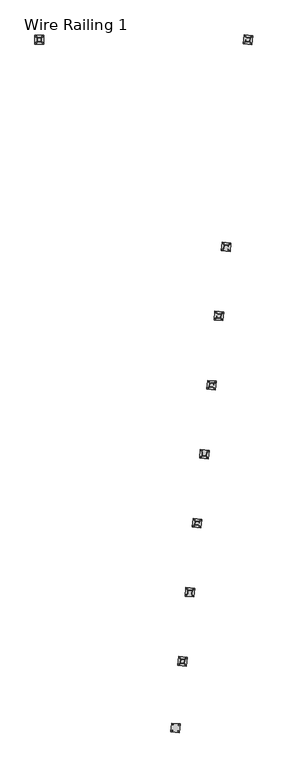
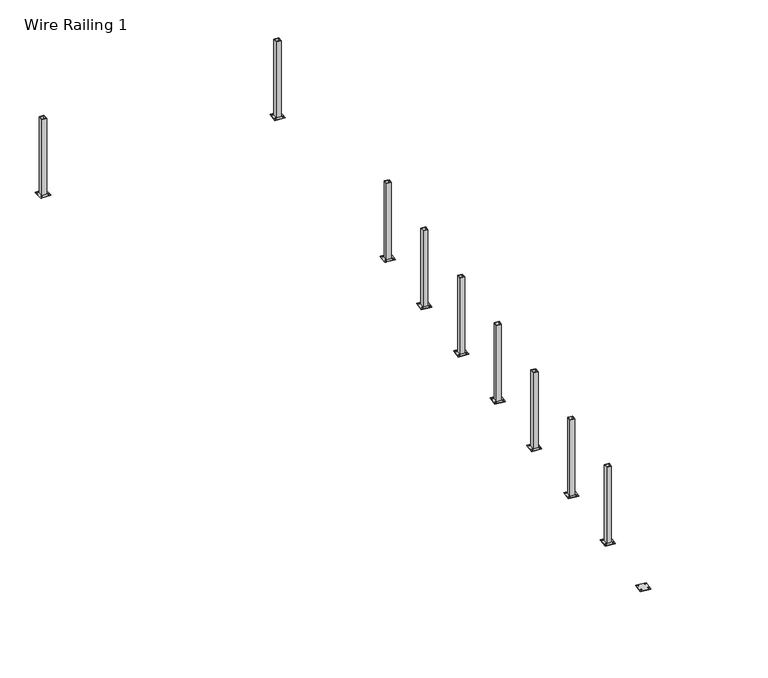
"""IFC4 building model written with IfcOpenShell, lengths in millimetres: railing geometry, Wire Railing 1."""

import ifcopenshell
import ifcopenshell.guid

model = None  # the IFC model being written
_history = None  # IfcOwnerHistory: only IFC2X3 demands one
_inside = {}  # id of a spatial element -> (the spatial element, [elements in it])
_under = {}  # id of a project, library or spatial element -> (it, [spatial elements below it])
_declared = {}  # id of a project -> (the project, [libraries it declares])
_typed = {}  # id of a type object -> (the type object, [elements of that type])
_made_of = {}  # id of a material, layer set ... -> (it, [elements and type objects made of it])


def new_model(schema):
    """Start an empty IFC model of exactly this schema.

    Asked for "IFC4X3", IfcOpenShell would pick the latest addendum, in which some entities
    have other attributes; the version numbers below select the first issue.
    IFC2X3 requires an IfcOwnerHistory on every rooted entity: one is made here for all.
    """
    global model, _history
    if schema == "IFC4X3":
        model = ifcopenshell.file(schema_version=(4, 3, 0, 0))
    else:
        model = ifcopenshell.file(schema=schema)
    _inside.clear()
    _under.clear()
    _declared.clear()
    _typed.clear()
    _made_of.clear()
    _history = None
    if model.schema == "IFC2X3":
        org = make("IfcOrganization", Name="unknown")
        user = make(
            "IfcPersonAndOrganization",
            ThePerson=make("IfcPerson", FamilyName="unknown"),
            TheOrganization=org,
        )
        app = make(
            "IfcApplication",
            ApplicationDeveloper=org,
            Version="unknown",
            ApplicationFullName="unknown",
            ApplicationIdentifier="unknown",
        )
        _history = make(
            "IfcOwnerHistory",
            OwningUser=user,
            OwningApplication=app,
            ChangeAction="ADDED",
            CreationDate=0,
        )
    return model


def make(cls, **values):
    """One entity of the class cls with the attributes given. An attribute that is None is left unset."""
    return model.create_entity(
        cls, **{name: value for name, value in values.items() if value is not None}
    )


def rooted(cls, **values):
    """An entity with a GlobalId (a new one), such as an element, a storey or a relation."""
    return make(cls, GlobalId=ifcopenshell.guid.new(), OwnerHistory=_history, **values)


def si_unit(unit_type, name, prefix=None):
    """IfcSIUnit, for example si_unit("LENGTHUNIT", "METRE", prefix="MILLI")."""
    return make("IfcSIUnit", UnitType=unit_type, Prefix=prefix, Name=name)


def assignment(units):
    """IfcUnitAssignment: the units of a project."""
    return None if units is None else make("IfcUnitAssignment", Units=units)


def point(xyz):
    """IfcCartesianPoint."""
    return None if xyz is None else make("IfcCartesianPoint", Coordinates=xyz)


def direction(xyz):
    """IfcDirection."""
    return None if xyz is None else make("IfcDirection", DirectionRatios=xyz)


def frame(location, z_axis=None, x_axis=None):
    """IfcAxis2Placement3D, a coordinate frame: its origin and axes. An axis left out is left unset."""
    return make(
        "IfcAxis2Placement3D",
        Location=point(location),
        Axis=direction(z_axis),
        RefDirection=direction(x_axis),
    )


def frame_2d(location, x_axis=None):
    """IfcAxis2Placement2D, a coordinate frame in the plane: its origin and x axis."""
    return make(
        "IfcAxis2Placement2D", Location=point(location), RefDirection=direction(x_axis)
    )


def origin():
    """The frame at (0, 0, 0) with its axes left unset."""
    return frame((0.0, 0.0, 0.0))


def place(relative_to, where):
    """IfcLocalPlacement: puts the frame where relative to a parent placement (None: the world)."""
    return make(
        "IfcLocalPlacement", PlacementRelTo=relative_to, RelativePlacement=where
    )


def context(
    kind, dimensions, precision=None, world=None, true_north=None, identifier=None
):
    """IfcGeometricRepresentationContext, for example the 3D "Model" context."""
    return make(
        "IfcGeometricRepresentationContext",
        ContextIdentifier=identifier,
        ContextType=kind,
        CoordinateSpaceDimension=dimensions,
        Precision=precision,
        WorldCoordinateSystem=world,
        TrueNorth=true_north,
    )


def project(units=None, contexts=None):
    """IfcProject with its units and contexts."""
    return rooted(
        "IfcProject",
        Name="project",
        RepresentationContexts=contexts,
        UnitsInContext=assignment(units),
    )


def spatial(cls, under=None, at=None, **own):
    """A site, building, storey or space (cls), placed at a placement, below another one or the project."""
    s = rooted(cls, ObjectPlacement=at, **own)
    if under is not None:
        _under.setdefault(under.id(), (under, []))[1].append(s)
    return s


def polyline(points):
    """IfcPolyline through the points."""
    return make("IfcPolyline", Points=[point(p) for p in points])


def circle_curve(where, radius):
    """IfcCircle in the frame where."""
    return make("IfcCircle", Position=where, Radius=radius)


def trimmed(basis, trim1, trim2, sense, master):
    """IfcTrimmedCurve: the piece of a basis curve between two trims."""
    return make(
        "IfcTrimmedCurve",
        BasisCurve=basis,
        Trim1=trim1,
        Trim2=trim2,
        SenseAgreement=sense,
        MasterRepresentation=master,
    )


def segment(curve, same_sense, transition):
    """IfcCompositeCurveSegment."""
    return make(
        "IfcCompositeCurveSegment",
        Transition=transition,
        SameSense=same_sense,
        ParentCurve=curve,
    )


def composite_curve(segments, self_intersect=None):
    """IfcCompositeCurve: segments joined end to end."""
    return make("IfcCompositeCurve", Segments=segments, SelfIntersect=self_intersect)


def outline(outer, holes=None, kind="AREA"):
    """IfcArbitraryClosedProfileDef: a profile drawn as a closed curve; with holes, ...WithVoids."""
    if holes is None:
        return make("IfcArbitraryClosedProfileDef", ProfileType=kind, OuterCurve=outer)
    return make(
        "IfcArbitraryProfileDefWithVoids",
        ProfileType=kind,
        OuterCurve=outer,
        InnerCurves=holes,
    )


def extrude(swept, where, along, depth):
    """IfcExtrudedAreaSolid: the profile swept, set in the frame where, extruded along a direction by depth."""
    return make(
        "IfcExtrudedAreaSolid",
        SweptArea=swept,
        Position=where,
        ExtrudedDirection=direction(along),
        Depth=depth,
    )


def shape(context_of_items, identifier, shape_type, items):
    """IfcShapeRepresentation: the items that make up one representation, for example the "Body"."""
    return make(
        "IfcShapeRepresentation",
        ContextOfItems=context_of_items,
        RepresentationIdentifier=identifier,
        RepresentationType=shape_type,
        Items=items,
    )


def source(mapping_origin, context_of_items, identifier, shape_type, items):
    """IfcRepresentationMap: a shape defined once, which mapped items show again and again."""
    return make(
        "IfcRepresentationMap",
        MappingOrigin=mapping_origin,
        MappedRepresentation=shape(context_of_items, identifier, shape_type, items),
    )


def transform(
    local_origin,
    x_axis=None,
    y_axis=None,
    z_axis=None,
    scale=None,
    scale2=None,
    scale3=None,
    uniform=True,
):
    """IfcCartesianTransformationOperator3D, or its non-uniform kind. x_axis, y_axis, z_axis: its Axis1, 2, 3."""
    if uniform:
        return make(
            "IfcCartesianTransformationOperator3D",
            Axis1=direction(x_axis),
            Axis2=direction(y_axis),
            LocalOrigin=point(local_origin),
            Scale=scale,
            Axis3=direction(z_axis),
        )
    return make(
        "IfcCartesianTransformationOperator3DnonUniform",
        Axis1=direction(x_axis),
        Axis2=direction(y_axis),
        LocalOrigin=point(local_origin),
        Scale=scale,
        Axis3=direction(z_axis),
        Scale2=scale2,
        Scale3=scale3,
    )


def mapped(mapping_source, mapping_target):
    """IfcMappedItem: shows the shape of a source again, moved by a transform."""
    return make(
        "IfcMappedItem", MappingSource=mapping_source, MappingTarget=mapping_target
    )


def made_of(thing, what):
    """Note that an element or type object is made of a material, layer set ...; save() writes the relation."""
    if what is not None:
        _made_of.setdefault(what.id(), (what, []))[1].append(thing)
    return thing


def element(
    cls,
    number,
    at=None,
    inside=None,
    cuts=None,
    type_object=None,
    material=None,
    context=None,
    identifier="Body",
    shape_type=None,
    held_by="IfcProductDefinitionShape",
    body=None,
    shapes=None,
    **own,
):
    """One element of the class cls, such as IfcWall. Its Tag is "e" and its number.

    at: its placement. inside: the storey or other place that contains it. cuts: it is an
    opening in that element (IfcRelVoidsElement). A single representation is given by context,
    identifier, shape_type and body (its items); several are given by shapes. held_by: the class
    of the entity that holds the representations. save() writes the other relations.
    """
    e = rooted(cls, Tag="e%d" % number, ObjectPlacement=at, **own)
    if body is not None:
        shapes = [shape(context, identifier, shape_type, body)]
    if shapes is not None:
        e.Representation = make(held_by, Representations=shapes)
    if inside is not None:
        _inside.setdefault(inside.id(), (inside, []))[1].append(e)
    if cuts is not None:
        rooted(
            "IfcRelVoidsElement", RelatingBuildingElement=cuts, RelatedOpeningElement=e
        )
    if type_object is not None:
        _typed.setdefault(type_object.id(), (type_object, []))[1].append(e)
    return made_of(e, material)


def aggregate(whole, parts):
    """IfcRelAggregates: a whole, such as a stair, and the parts it consists of."""
    return rooted("IfcRelAggregates", RelatingObject=whole, RelatedObjects=parts)


def save(model, path):
    """Write the relations noted so far, then the file.

    IfcRelAggregates (storeys below a building ...), IfcRelContainedInSpatialStructure (elements
    in a storey), IfcRelDefinesByType, IfcRelAssociatesMaterial and IfcRelDeclares: one each for
    every whole, place, type object, material and project.
    """
    for whole, parts in _under.values():
        aggregate(whole, parts)
    for where, things in _inside.values():
        rooted(
            "IfcRelContainedInSpatialStructure",
            RelatedElements=things,
            RelatingStructure=where,
        )
    for kind, things in _typed.values():
        rooted("IfcRelDefinesByType", RelatedObjects=things, RelatingType=kind)
    for what, things in _made_of.values():
        rooted("IfcRelAssociatesMaterial", RelatedObjects=things, RelatingMaterial=what)
    for by, libraries in _declared.values():
        rooted("IfcRelDeclares", RelatingContext=by, RelatedDefinitions=libraries)
    model.write(path)


def wire_railing_1_b7aef56b(model_context):
    return source(origin(), model_context, "Body", "SweptSolid", [
        extrude(outline(composite_curve([segment(trimmed(circle_curve(frame_2d((34964.0191905, 37829.4240871)), 6.35), [point((34957.7039765, 37830.0878428))], [point((34970.3344045, 37828.7603313))], False, "CARTESIAN"), True, "CONTINUOUS"), segment(trimmed(circle_curve(frame_2d((34964.0191905, 37829.4240871)), 6.35), [point((34970.3344045, 37828.7603313))], [point((34957.7039765, 37830.0878428))], False, "CARTESIAN"), True, "CONTINUOUS")], self_intersect=False)), frame((0.0, 0.0, 269259.05), z_axis=(0.0, 0.0, 1.0), x_axis=(1.0, 0.0, 0.0)), (0.0, 0.0, 1.0), 12.7),
        extrude(outline(composite_curve([segment(trimmed(circle_curve(frame_2d((35052.432187, 37820.1315067)), 6.35), [point((35046.116973, 37820.7952624))], [point((35058.747401, 37819.4677509))], False, "CARTESIAN"), True, "CONTINUOUS"), segment(trimmed(circle_curve(frame_2d((35052.432187, 37820.1315067)), 6.35), [point((35058.747401, 37819.4677509))], [point((35046.116973, 37820.7952624))], False, "CARTESIAN"), True, "CONTINUOUS")], self_intersect=False)), frame((0.0, 0.0, 269259.05), z_axis=(0.0, 0.0, 1.0), x_axis=(1.0, 0.0, 0.0)), (0.0, 0.0, 1.0), 12.7),
        extrude(outline(composite_curve([segment(trimmed(circle_curve(frame_2d((34973.3117709, 37917.8370836)), 6.35), [point((34966.9965569, 37918.5008393))], [point((34979.6269849, 37917.1733278))], False, "CARTESIAN"), True, "CONTINUOUS"), segment(trimmed(circle_curve(frame_2d((34973.3117709, 37917.8370836)), 6.35), [point((34979.6269849, 37917.1733278))], [point((34966.9965569, 37918.5008393))], False, "CARTESIAN"), True, "CONTINUOUS")], self_intersect=False)), frame((0.0, 0.0, 269259.05), z_axis=(0.0, 0.0, 1.0), x_axis=(1.0, 0.0, 0.0)), (0.0, 0.0, 1.0), 12.7),
        extrude(outline(composite_curve([segment(trimmed(circle_curve(frame_2d((35061.7247674, 37908.5445032)), 6.35), [point((35055.4095533, 37909.2082589))], [point((35068.0399814, 37907.8807474))], False, "CARTESIAN"), True, "CONTINUOUS"), segment(trimmed(circle_curve(frame_2d((35061.7247674, 37908.5445032)), 6.35), [point((35068.0399814, 37907.8807474))], [point((35055.4095533, 37909.2082589))], False, "CARTESIAN"), True, "CONTINUOUS")], self_intersect=False)), frame((0.0, 0.0, 269259.05), z_axis=(0.0, 0.0, 1.0), x_axis=(1.0, 0.0, 0.0)), (0.0, 0.0, 1.0), 12.7),
        extrude(outline(polyline([(35069.3865619, 37799.1945973), (34943.0822812, 37812.4697122), (34956.357396, 37938.7739929), (35082.6616767, 37925.498878), (35069.3865619, 37799.1945973)])), frame((0.0, 0.0, 269259.05), z_axis=(0.0, 0.0, 1.0), x_axis=(1.0, 0.0, 0.0)), (0.0, 0.0, 1.0), 6.35),
        extrude(outline(polyline([(35039.7164058, 37835.8341887), (34979.7218725, 37842.1398682), (34986.027552, 37902.1344016), (35046.0220854, 37895.828722), (35039.7164058, 37835.8341887)]), holes=[polyline([(35034.0649475, 37842.8131584), (35039.0431156, 37890.1772637), (34991.6790103, 37895.1554318), (34986.7008423, 37847.7913265), (35034.0649475, 37842.8131584)])]), frame((0.0, 0.0, 269259.05), z_axis=(0.0, 0.0, 1.0), x_axis=(1.0, 0.0, 0.0)), (0.0, 0.0, 1.0), 1047.75),
        extrude(outline(composite_curve([segment(trimmed(circle_curve(frame_2d((34858.2648202, 36823.238465)), 6.35), [point((34851.9496061, 36823.9022208))], [point((34864.5800342, 36822.5747093))], False, "CARTESIAN"), True, "CONTINUOUS"), segment(trimmed(circle_curve(frame_2d((34858.2648202, 36823.238465)), 6.35), [point((34864.5800342, 36822.5747093))], [point((34851.9496061, 36823.9022208))], False, "CARTESIAN"), True, "CONTINUOUS")], self_intersect=False)), frame((0.0, 0.0, 269259.05), z_axis=(0.0, 0.0, 1.0), x_axis=(1.0, 0.0, 0.0)), (0.0, 0.0, 1.0), 12.7),
        extrude(outline(composite_curve([segment(trimmed(circle_curve(frame_2d((34946.6778167, 36813.9458846)), 6.35), [point((34940.3626026, 36814.6096404))], [point((34952.9930307, 36813.2821289))], False, "CARTESIAN"), True, "CONTINUOUS"), segment(trimmed(circle_curve(frame_2d((34946.6778167, 36813.9458846)), 6.35), [point((34952.9930307, 36813.2821289))], [point((34940.3626026, 36814.6096404))], False, "CARTESIAN"), True, "CONTINUOUS")], self_intersect=False)), frame((0.0, 0.0, 269259.05), z_axis=(0.0, 0.0, 1.0), x_axis=(1.0, 0.0, 0.0)), (0.0, 0.0, 1.0), 12.7),
        extrude(outline(composite_curve([segment(trimmed(circle_curve(frame_2d((34867.5574005, 36911.6514615)), 6.35), [point((34861.2421865, 36912.3152173))], [point((34873.8726146, 36910.9877058))], False, "CARTESIAN"), True, "CONTINUOUS"), segment(trimmed(circle_curve(frame_2d((34867.5574005, 36911.6514615)), 6.35), [point((34873.8726146, 36910.9877058))], [point((34861.2421865, 36912.3152173))], False, "CARTESIAN"), True, "CONTINUOUS")], self_intersect=False)), frame((0.0, 0.0, 269259.05), z_axis=(0.0, 0.0, 1.0), x_axis=(1.0, 0.0, 0.0)), (0.0, 0.0, 1.0), 12.7),
        extrude(outline(composite_curve([segment(trimmed(circle_curve(frame_2d((34955.970397, 36902.3588811)), 6.35), [point((34949.655183, 36903.0226369))], [point((34962.2856111, 36901.6951254))], False, "CARTESIAN"), True, "CONTINUOUS"), segment(trimmed(circle_curve(frame_2d((34955.970397, 36902.3588811)), 6.35), [point((34962.2856111, 36901.6951254))], [point((34949.655183, 36903.0226369))], False, "CARTESIAN"), True, "CONTINUOUS")], self_intersect=False)), frame((0.0, 0.0, 269259.05), z_axis=(0.0, 0.0, 1.0), x_axis=(1.0, 0.0, 0.0)), (0.0, 0.0, 1.0), 12.7),
        extrude(outline(polyline([(34963.6321915, 36793.0089753), (34837.3279108, 36806.2840901), (34850.6030257, 36932.5883709), (34976.9073064, 36919.313256), (34963.6321915, 36793.0089753)])), frame((0.0, 0.0, 269259.05), z_axis=(0.0, 0.0, 1.0), x_axis=(1.0, 0.0, 0.0)), (0.0, 0.0, 1.0), 6.35),
        extrude(outline(polyline([(34933.9620355, 36829.6485666), (34873.9675022, 36835.9542462), (34880.2731817, 36895.9487795), (34940.267715, 36889.6431), (34933.9620355, 36829.6485666)]), holes=[polyline([(34928.3105772, 36836.6275364), (34933.2887453, 36883.9916417), (34885.92464, 36888.9698097), (34880.9464719, 36841.6057045), (34928.3105772, 36836.6275364)])]), frame((0.0, 0.0, 269259.05), z_axis=(0.0, 0.0, 1.0), x_axis=(1.0, 0.0, 0.0)), (0.0, 0.0, 1.0), 1047.75),
        extrude(outline(composite_curve([segment(trimmed(circle_curve(frame_2d((34752.5104498, 35817.052843)), 6.35), [point((34746.1952358, 35817.7165987))], [point((34758.8256639, 35816.3890873))], False, "CARTESIAN"), True, "CONTINUOUS"), segment(trimmed(circle_curve(frame_2d((34752.5104498, 35817.052843)), 6.35), [point((34758.8256639, 35816.3890873))], [point((34746.1952358, 35817.7165987))], False, "CARTESIAN"), True, "CONTINUOUS")], self_intersect=False)), frame((0.0, 0.0, 269259.05), z_axis=(0.0, 0.0, 1.0), x_axis=(1.0, 0.0, 0.0)), (0.0, 0.0, 1.0), 12.7),
        extrude(outline(composite_curve([segment(trimmed(circle_curve(frame_2d((34840.9234463, 35807.7602626)), 6.35), [point((34834.6082323, 35808.4240184))], [point((34847.2386604, 35807.0965069))], False, "CARTESIAN"), True, "CONTINUOUS"), segment(trimmed(circle_curve(frame_2d((34840.9234463, 35807.7602626)), 6.35), [point((34847.2386604, 35807.0965069))], [point((34834.6082323, 35808.4240184))], False, "CARTESIAN"), True, "CONTINUOUS")], self_intersect=False)), frame((0.0, 0.0, 269259.05), z_axis=(0.0, 0.0, 1.0), x_axis=(1.0, 0.0, 0.0)), (0.0, 0.0, 1.0), 12.7),
        extrude(outline(composite_curve([segment(trimmed(circle_curve(frame_2d((34761.8030302, 35905.4658395)), 6.35), [point((34755.4878162, 35906.1295952))], [point((34768.1182442, 35904.8020838))], False, "CARTESIAN"), True, "CONTINUOUS"), segment(trimmed(circle_curve(frame_2d((34761.8030302, 35905.4658395)), 6.35), [point((34768.1182442, 35904.8020838))], [point((34755.4878162, 35906.1295952))], False, "CARTESIAN"), True, "CONTINUOUS")], self_intersect=False)), frame((0.0, 0.0, 269259.05), z_axis=(0.0, 0.0, 1.0), x_axis=(1.0, 0.0, 0.0)), (0.0, 0.0, 1.0), 12.7),
        extrude(outline(composite_curve([segment(trimmed(circle_curve(frame_2d((34850.2160267, 35896.1732591)), 6.35), [point((34843.9008127, 35896.8370148))], [point((34856.5312407, 35895.5095034))], False, "CARTESIAN"), True, "CONTINUOUS"), segment(trimmed(circle_curve(frame_2d((34850.2160267, 35896.1732591)), 6.35), [point((34856.5312407, 35895.5095034))], [point((34843.9008127, 35896.8370148))], False, "CARTESIAN"), True, "CONTINUOUS")], self_intersect=False)), frame((0.0, 0.0, 269259.05), z_axis=(0.0, 0.0, 1.0), x_axis=(1.0, 0.0, 0.0)), (0.0, 0.0, 1.0), 12.7),
        extrude(outline(polyline([(34857.8778212, 35786.8233533), (34731.5735405, 35800.0984681), (34744.8486553, 35926.4027488), (34871.152936, 35913.127634), (34857.8778212, 35786.8233533)])), frame((0.0, 0.0, 269259.05), z_axis=(0.0, 0.0, 1.0), x_axis=(1.0, 0.0, 0.0)), (0.0, 0.0, 1.0), 6.35),
        extrude(outline(polyline([(34828.2076652, 35823.4629446), (34768.2131318, 35829.7686242), (34774.5188114, 35889.7631575), (34834.5133447, 35883.4574779), (34828.2076652, 35823.4629446)]), holes=[polyline([(34822.5562069, 35830.4419144), (34827.5343749, 35877.8060197), (34780.1702697, 35882.7841877), (34775.1921016, 35835.4200824), (34822.5562069, 35830.4419144)])]), frame((0.0, 0.0, 269259.05), z_axis=(0.0, 0.0, 1.0), x_axis=(1.0, 0.0, 0.0)), (0.0, 0.0, 1.0), 1047.75),
        extrude(outline(composite_curve([segment(trimmed(circle_curve(frame_2d((34646.7560795, 34810.867221)), 6.35), [point((34640.4408654, 34811.5309767))], [point((34653.0712935, 34810.2034652))], False, "CARTESIAN"), True, "CONTINUOUS"), segment(trimmed(circle_curve(frame_2d((34646.7560795, 34810.867221)), 6.35), [point((34653.0712935, 34810.2034652))], [point((34640.4408654, 34811.5309767))], False, "CARTESIAN"), True, "CONTINUOUS")], self_intersect=False)), frame((0.0, 0.0, 269259.05), z_axis=(0.0, 0.0, 1.0), x_axis=(1.0, 0.0, 0.0)), (0.0, 0.0, 1.0), 12.7),
        extrude(outline(composite_curve([segment(trimmed(circle_curve(frame_2d((34735.169076, 34801.5746406)), 6.35), [point((34728.8538619, 34802.2383963))], [point((34741.48429, 34800.9108848))], False, "CARTESIAN"), True, "CONTINUOUS"), segment(trimmed(circle_curve(frame_2d((34735.169076, 34801.5746406)), 6.35), [point((34741.48429, 34800.9108848))], [point((34728.8538619, 34802.2383963))], False, "CARTESIAN"), True, "CONTINUOUS")], self_intersect=False)), frame((0.0, 0.0, 269259.05), z_axis=(0.0, 0.0, 1.0), x_axis=(1.0, 0.0, 0.0)), (0.0, 0.0, 1.0), 12.7),
        extrude(outline(composite_curve([segment(trimmed(circle_curve(frame_2d((34656.0486599, 34899.2802175)), 6.35), [point((34649.7334458, 34899.9439732))], [point((34662.3638739, 34898.6164617))], False, "CARTESIAN"), True, "CONTINUOUS"), segment(trimmed(circle_curve(frame_2d((34656.0486599, 34899.2802175)), 6.35), [point((34662.3638739, 34898.6164617))], [point((34649.7334458, 34899.9439732))], False, "CARTESIAN"), True, "CONTINUOUS")], self_intersect=False)), frame((0.0, 0.0, 269259.05), z_axis=(0.0, 0.0, 1.0), x_axis=(1.0, 0.0, 0.0)), (0.0, 0.0, 1.0), 12.7),
        extrude(outline(composite_curve([segment(trimmed(circle_curve(frame_2d((34744.4616564, 34889.9876371)), 6.35), [point((34738.1464423, 34890.6513928))], [point((34750.7768704, 34889.3238813))], False, "CARTESIAN"), True, "CONTINUOUS"), segment(trimmed(circle_curve(frame_2d((34744.4616564, 34889.9876371)), 6.35), [point((34750.7768704, 34889.3238813))], [point((34738.1464423, 34890.6513928))], False, "CARTESIAN"), True, "CONTINUOUS")], self_intersect=False)), frame((0.0, 0.0, 269259.05), z_axis=(0.0, 0.0, 1.0), x_axis=(1.0, 0.0, 0.0)), (0.0, 0.0, 1.0), 12.7),
        extrude(outline(polyline([(34752.1234509, 34780.6377312), (34625.8191702, 34793.9128461), (34639.094285, 34920.2171268), (34765.3985657, 34906.942012), (34752.1234509, 34780.6377312)])), frame((0.0, 0.0, 269259.05), z_axis=(0.0, 0.0, 1.0), x_axis=(1.0, 0.0, 0.0)), (0.0, 0.0, 1.0), 6.35),
        extrude(outline(polyline([(34722.4532948, 34817.2773226), (34662.4587615, 34823.5830021), (34668.764441, 34883.5775355), (34728.7589744, 34877.2718559), (34722.4532948, 34817.2773226)]), holes=[polyline([(34716.8018365, 34824.2562924), (34721.7800046, 34871.6203976), (34674.4158993, 34876.5985657), (34669.4377313, 34829.2344604), (34716.8018365, 34824.2562924)])]), frame((0.0, 0.0, 269259.05), z_axis=(0.0, 0.0, 1.0), x_axis=(1.0, 0.0, 0.0)), (0.0, 0.0, 1.0), 1047.75),
        extrude(outline(composite_curve([segment(trimmed(circle_curve(frame_2d((34541.0017091, 33804.6815989)), 6.35), [point((34534.6864951, 33805.3453547))], [point((34547.3169232, 33804.0178432))], False, "CARTESIAN"), True, "CONTINUOUS"), segment(trimmed(circle_curve(frame_2d((34541.0017091, 33804.6815989)), 6.35), [point((34547.3169232, 33804.0178432))], [point((34534.6864951, 33805.3453547))], False, "CARTESIAN"), True, "CONTINUOUS")], self_intersect=False)), frame((0.0, 0.0, 269259.05), z_axis=(0.0, 0.0, 1.0), x_axis=(1.0, 0.0, 0.0)), (0.0, 0.0, 1.0), 12.7),
        extrude(outline(composite_curve([segment(trimmed(circle_curve(frame_2d((34629.4147056, 33795.3890186)), 6.35), [point((34623.0994916, 33796.0527743))], [point((34635.7299197, 33794.7252628))], False, "CARTESIAN"), True, "CONTINUOUS"), segment(trimmed(circle_curve(frame_2d((34629.4147056, 33795.3890186)), 6.35), [point((34635.7299197, 33794.7252628))], [point((34623.0994916, 33796.0527743))], False, "CARTESIAN"), True, "CONTINUOUS")], self_intersect=False)), frame((0.0, 0.0, 269259.05), z_axis=(0.0, 0.0, 1.0), x_axis=(1.0, 0.0, 0.0)), (0.0, 0.0, 1.0), 12.7),
        extrude(outline(composite_curve([segment(trimmed(circle_curve(frame_2d((34550.2942895, 33893.0945954)), 6.35), [point((34543.9790755, 33893.7583512))], [point((34556.6095036, 33892.4308397))], False, "CARTESIAN"), True, "CONTINUOUS"), segment(trimmed(circle_curve(frame_2d((34550.2942895, 33893.0945954)), 6.35), [point((34556.6095036, 33892.4308397))], [point((34543.9790755, 33893.7583512))], False, "CARTESIAN"), True, "CONTINUOUS")], self_intersect=False)), frame((0.0, 0.0, 269259.05), z_axis=(0.0, 0.0, 1.0), x_axis=(1.0, 0.0, 0.0)), (0.0, 0.0, 1.0), 12.7),
        extrude(outline(composite_curve([segment(trimmed(circle_curve(frame_2d((34638.707286, 33883.802015)), 6.35), [point((34632.392072, 33884.4657708))], [point((34645.0225001, 33883.1382593))], False, "CARTESIAN"), True, "CONTINUOUS"), segment(trimmed(circle_curve(frame_2d((34638.707286, 33883.802015)), 6.35), [point((34645.0225001, 33883.1382593))], [point((34632.392072, 33884.4657708))], False, "CARTESIAN"), True, "CONTINUOUS")], self_intersect=False)), frame((0.0, 0.0, 269259.05), z_axis=(0.0, 0.0, 1.0), x_axis=(1.0, 0.0, 0.0)), (0.0, 0.0, 1.0), 12.7),
        extrude(outline(polyline([(34646.3690805, 33774.4521092), (34520.0647998, 33787.7272241), (34533.3399146, 33914.0315048), (34659.6441954, 33900.7563899), (34646.3690805, 33774.4521092)])), frame((0.0, 0.0, 269259.05), z_axis=(0.0, 0.0, 1.0), x_axis=(1.0, 0.0, 0.0)), (0.0, 0.0, 1.0), 6.35),
        extrude(outline(polyline([(34616.6989245, 33811.0917005), (34556.7043911, 33817.3973801), (34563.0100707, 33877.3919134), (34623.004604, 33871.0862339), (34616.6989245, 33811.0917005)]), holes=[polyline([(34611.0474662, 33818.0706703), (34616.0256343, 33865.4347756), (34568.661529, 33870.4129437), (34563.6833609, 33823.0488384), (34611.0474662, 33818.0706703)])]), frame((0.0, 0.0, 269259.05), z_axis=(0.0, 0.0, 1.0), x_axis=(1.0, 0.0, 0.0)), (0.0, 0.0, 1.0), 1047.75),
        extrude(outline(composite_curve([segment(trimmed(circle_curve(frame_2d((34435.2473388, 32798.4959769)), 6.35), [point((34428.9321248, 32799.1597326))], [point((34441.5625528, 32797.8322212))], False, "CARTESIAN"), True, "CONTINUOUS"), segment(trimmed(circle_curve(frame_2d((34435.2473388, 32798.4959769)), 6.35), [point((34441.5625528, 32797.8322212))], [point((34428.9321248, 32799.1597326))], False, "CARTESIAN"), True, "CONTINUOUS")], self_intersect=False)), frame((0.0, 0.0, 269259.05), z_axis=(0.0, 0.0, 1.0), x_axis=(1.0, 0.0, 0.0)), (0.0, 0.0, 1.0), 12.7),
        extrude(outline(composite_curve([segment(trimmed(circle_curve(frame_2d((34523.6603353, 32789.2033965)), 6.35), [point((34517.3451213, 32789.8671523))], [point((34529.9755493, 32788.5396408))], False, "CARTESIAN"), True, "CONTINUOUS"), segment(trimmed(circle_curve(frame_2d((34523.6603353, 32789.2033965)), 6.35), [point((34529.9755493, 32788.5396408))], [point((34517.3451213, 32789.8671523))], False, "CARTESIAN"), True, "CONTINUOUS")], self_intersect=False)), frame((0.0, 0.0, 269259.05), z_axis=(0.0, 0.0, 1.0), x_axis=(1.0, 0.0, 0.0)), (0.0, 0.0, 1.0), 12.7),
        extrude(outline(composite_curve([segment(trimmed(circle_curve(frame_2d((34444.5399192, 32886.9089734)), 6.35), [point((34438.2247052, 32887.5727291))], [point((34450.8551332, 32886.2452177))], False, "CARTESIAN"), True, "CONTINUOUS"), segment(trimmed(circle_curve(frame_2d((34444.5399192, 32886.9089734)), 6.35), [point((34450.8551332, 32886.2452177))], [point((34438.2247052, 32887.5727291))], False, "CARTESIAN"), True, "CONTINUOUS")], self_intersect=False)), frame((0.0, 0.0, 269259.05), z_axis=(0.0, 0.0, 1.0), x_axis=(1.0, 0.0, 0.0)), (0.0, 0.0, 1.0), 12.7),
        extrude(outline(composite_curve([segment(trimmed(circle_curve(frame_2d((34532.9529157, 32877.616393)), 6.35), [point((34526.6377017, 32878.2801488))], [point((34539.2681297, 32876.9526373))], False, "CARTESIAN"), True, "CONTINUOUS"), segment(trimmed(circle_curve(frame_2d((34532.9529157, 32877.616393)), 6.35), [point((34539.2681297, 32876.9526373))], [point((34526.6377017, 32878.2801488))], False, "CARTESIAN"), True, "CONTINUOUS")], self_intersect=False)), frame((0.0, 0.0, 269259.05), z_axis=(0.0, 0.0, 1.0), x_axis=(1.0, 0.0, 0.0)), (0.0, 0.0, 1.0), 12.7),
        extrude(outline(polyline([(34540.6147102, 32768.2664872), (34414.3104295, 32781.541602), (34427.5855443, 32907.8458827), (34553.889825, 32894.5707679), (34540.6147102, 32768.2664872)])), frame((0.0, 0.0, 269259.05), z_axis=(0.0, 0.0, 1.0), x_axis=(1.0, 0.0, 0.0)), (0.0, 0.0, 1.0), 6.35),
        extrude(outline(polyline([(34510.9445541, 32804.9060785), (34450.9500208, 32811.2117581), (34457.2557004, 32871.2062914), (34517.2502337, 32864.9006119), (34510.9445541, 32804.9060785)]), holes=[polyline([(34505.2930959, 32811.8850483), (34510.2712639, 32859.2491536), (34462.9071586, 32864.2273216), (34457.9289906, 32816.8632164), (34505.2930959, 32811.8850483)])]), frame((0.0, 0.0, 269259.05), z_axis=(0.0, 0.0, 1.0), x_axis=(1.0, 0.0, 0.0)), (0.0, 0.0, 1.0), 1047.75),
        extrude(outline(composite_curve([segment(trimmed(circle_curve(frame_2d((34329.4929685, 31792.3103549)), 6.35), [point((34323.1777544, 31792.9741106))], [point((34335.8081825, 31791.6465991))], False, "CARTESIAN"), True, "CONTINUOUS"), segment(trimmed(circle_curve(frame_2d((34329.4929685, 31792.3103549)), 6.35), [point((34335.8081825, 31791.6465991))], [point((34323.1777544, 31792.9741106))], False, "CARTESIAN"), True, "CONTINUOUS")], self_intersect=False)), frame((0.0, 0.0, 269259.05), z_axis=(0.0, 0.0, 1.0), x_axis=(1.0, 0.0, 0.0)), (0.0, 0.0, 1.0), 12.7),
        extrude(outline(composite_curve([segment(trimmed(circle_curve(frame_2d((34417.905965, 31783.0177745)), 6.35), [point((34411.5907509, 31783.6815302))], [point((34424.221179, 31782.3540188))], False, "CARTESIAN"), True, "CONTINUOUS"), segment(trimmed(circle_curve(frame_2d((34417.905965, 31783.0177745)), 6.35), [point((34424.221179, 31782.3540188))], [point((34411.5907509, 31783.6815302))], False, "CARTESIAN"), True, "CONTINUOUS")], self_intersect=False)), frame((0.0, 0.0, 269259.05), z_axis=(0.0, 0.0, 1.0), x_axis=(1.0, 0.0, 0.0)), (0.0, 0.0, 1.0), 12.7),
        extrude(outline(composite_curve([segment(trimmed(circle_curve(frame_2d((34338.7855489, 31880.7233514)), 6.35), [point((34332.4703348, 31881.3871071))], [point((34345.1007629, 31880.0595956))], False, "CARTESIAN"), True, "CONTINUOUS"), segment(trimmed(circle_curve(frame_2d((34338.7855489, 31880.7233514)), 6.35), [point((34345.1007629, 31880.0595956))], [point((34332.4703348, 31881.3871071))], False, "CARTESIAN"), True, "CONTINUOUS")], self_intersect=False)), frame((0.0, 0.0, 269259.05), z_axis=(0.0, 0.0, 1.0), x_axis=(1.0, 0.0, 0.0)), (0.0, 0.0, 1.0), 12.7),
        extrude(outline(composite_curve([segment(trimmed(circle_curve(frame_2d((34427.1985454, 31871.430771)), 6.35), [point((34420.8833313, 31872.0945267))], [point((34433.5137594, 31870.7670152))], False, "CARTESIAN"), True, "CONTINUOUS"), segment(trimmed(circle_curve(frame_2d((34427.1985454, 31871.430771)), 6.35), [point((34433.5137594, 31870.7670152))], [point((34420.8833313, 31872.0945267))], False, "CARTESIAN"), True, "CONTINUOUS")], self_intersect=False)), frame((0.0, 0.0, 269259.05), z_axis=(0.0, 0.0, 1.0), x_axis=(1.0, 0.0, 0.0)), (0.0, 0.0, 1.0), 12.7),
        extrude(outline(polyline([(34434.8603398, 31762.0808652), (34308.5560591, 31775.35598), (34321.831174, 31901.6602607), (34448.1354547, 31888.3851459), (34434.8603398, 31762.0808652)])), frame((0.0, 0.0, 269259.05), z_axis=(0.0, 0.0, 1.0), x_axis=(1.0, 0.0, 0.0)), (0.0, 0.0, 1.0), 6.35),
        extrude(outline(polyline([(34405.1901838, 31798.7204565), (34345.1956505, 31805.026136), (34351.50133, 31865.0206694), (34411.4958634, 31858.7149898), (34405.1901838, 31798.7204565)]), holes=[polyline([(34399.5387255, 31805.6994263), (34404.5168936, 31853.0635315), (34357.1527883, 31858.0416996), (34352.1746202, 31810.6775943), (34399.5387255, 31805.6994263)])]), frame((0.0, 0.0, 269259.05), z_axis=(0.0, 0.0, 1.0), x_axis=(1.0, 0.0, 0.0)), (0.0, 0.0, 1.0), 1047.75),
        extrude(outline(composite_curve([segment(trimmed(circle_curve(frame_2d((35281.2823015, 40847.9809531)), 6.35), [point((35274.9670875, 40848.6447089))], [point((35287.5975156, 40847.3171974))], False, "CARTESIAN"), True, "CONTINUOUS"), segment(trimmed(circle_curve(frame_2d((35281.2823015, 40847.9809531)), 6.35), [point((35287.5975156, 40847.3171974))], [point((35274.9670875, 40848.6447089))], False, "CARTESIAN"), True, "CONTINUOUS")], self_intersect=False)), frame((0.0, 0.0, 269259.05), z_axis=(0.0, 0.0, 1.0), x_axis=(1.0, 0.0, 0.0)), (0.0, 0.0, 1.0), 12.7),
        extrude(outline(composite_curve([segment(trimmed(circle_curve(frame_2d((35369.695298, 40838.6883728)), 6.35), [point((35363.380084, 40839.3521285))], [point((35376.0105121, 40838.024617))], False, "CARTESIAN"), True, "CONTINUOUS"), segment(trimmed(circle_curve(frame_2d((35369.695298, 40838.6883728)), 6.35), [point((35376.0105121, 40838.024617))], [point((35363.380084, 40839.3521285))], False, "CARTESIAN"), True, "CONTINUOUS")], self_intersect=False)), frame((0.0, 0.0, 269259.05), z_axis=(0.0, 0.0, 1.0), x_axis=(1.0, 0.0, 0.0)), (0.0, 0.0, 1.0), 12.7),
        extrude(outline(composite_curve([segment(trimmed(circle_curve(frame_2d((35290.5748819, 40936.3939496)), 6.35), [point((35284.2596679, 40937.0577054))], [point((35296.8900959, 40935.7301939))], False, "CARTESIAN"), True, "CONTINUOUS"), segment(trimmed(circle_curve(frame_2d((35290.5748819, 40936.3939496)), 6.35), [point((35296.8900959, 40935.7301939))], [point((35284.2596679, 40937.0577054))], False, "CARTESIAN"), True, "CONTINUOUS")], self_intersect=False)), frame((0.0, 0.0, 269259.05), z_axis=(0.0, 0.0, 1.0), x_axis=(1.0, 0.0, 0.0)), (0.0, 0.0, 1.0), 12.7),
        extrude(outline(composite_curve([segment(trimmed(circle_curve(frame_2d((35378.9878784, 40927.1013693)), 6.35), [point((35372.6726644, 40927.765125))], [point((35385.3030924, 40926.4376135))], False, "CARTESIAN"), True, "CONTINUOUS"), segment(trimmed(circle_curve(frame_2d((35378.9878784, 40927.1013693)), 6.35), [point((35385.3030924, 40926.4376135))], [point((35372.6726644, 40927.765125))], False, "CARTESIAN"), True, "CONTINUOUS")], self_intersect=False)), frame((0.0, 0.0, 269259.05), z_axis=(0.0, 0.0, 1.0), x_axis=(1.0, 0.0, 0.0)), (0.0, 0.0, 1.0), 12.7),
        extrude(outline(polyline([(35386.6496729, 40817.7514634), (35260.3453922, 40831.0265783), (35273.620507, 40957.330859), (35399.9247877, 40944.0557441), (35386.6496729, 40817.7514634)])), frame((0.0, 0.0, 269259.05), z_axis=(0.0, 0.0, 1.0), x_axis=(1.0, 0.0, 0.0)), (0.0, 0.0, 1.0), 6.35),
        extrude(outline(polyline([(35356.9795169, 40854.3910548), (35296.9849835, 40860.6967343), (35303.2906631, 40920.6912676), (35363.2851964, 40914.3855881), (35356.9795169, 40854.3910548)]), holes=[polyline([(35351.3280586, 40861.3700245), (35356.3062266, 40908.7341298), (35308.9421214, 40913.7122979), (35303.9639533, 40866.3481926), (35351.3280586, 40861.3700245)])]), frame((0.0, 0.0, 269259.05), z_axis=(0.0, 0.0, 1.0), x_axis=(1.0, 0.0, 0.0)), (0.0, 0.0, 1.0), 1047.75),
        extrude(outline(composite_curve([segment(trimmed(circle_curve(frame_2d((32337.1627201, 40843.0911612)), 6.35), [point((32337.1627201, 40836.7411612))], [point((32337.1627201, 40849.4411612))], False, "CARTESIAN"), True, "CONTINUOUS"), segment(trimmed(circle_curve(frame_2d((32337.1627201, 40843.0911612)), 6.35), [point((32337.1627201, 40849.4411612))], [point((32337.1627201, 40836.7411612))], False, "CARTESIAN"), True, "CONTINUOUS")], self_intersect=False)), frame((0.0, 0.0, 269259.05), z_axis=(0.0, 0.0, 1.0), x_axis=(1.0, 0.0, 0.0)), (0.0, 0.0, 1.0), 12.7),
        extrude(outline(composite_curve([segment(trimmed(circle_curve(frame_2d((32337.1627201, 40931.9911612)), 6.35), [point((32337.1627201, 40925.6411612))], [point((32337.1627201, 40938.3411612))], False, "CARTESIAN"), True, "CONTINUOUS"), segment(trimmed(circle_curve(frame_2d((32337.1627201, 40931.9911612)), 6.35), [point((32337.1627201, 40938.3411612))], [point((32337.1627201, 40925.6411612))], False, "CARTESIAN"), True, "CONTINUOUS")], self_intersect=False)), frame((0.0, 0.0, 269259.05), z_axis=(0.0, 0.0, 1.0), x_axis=(1.0, 0.0, 0.0)), (0.0, 0.0, 1.0), 12.7),
        extrude(outline(composite_curve([segment(trimmed(circle_curve(frame_2d((32248.2627201, 40843.0911612)), 6.35), [point((32248.2627201, 40836.7411612))], [point((32248.2627201, 40849.4411612))], False, "CARTESIAN"), True, "CONTINUOUS"), segment(trimmed(circle_curve(frame_2d((32248.2627201, 40843.0911612)), 6.35), [point((32248.2627201, 40849.4411612))], [point((32248.2627201, 40836.7411612))], False, "CARTESIAN"), True, "CONTINUOUS")], self_intersect=False)), frame((0.0, 0.0, 269259.05), z_axis=(0.0, 0.0, 1.0), x_axis=(1.0, 0.0, 0.0)), (0.0, 0.0, 1.0), 12.7),
        extrude(outline(composite_curve([segment(trimmed(circle_curve(frame_2d((32248.2627201, 40931.9911612)), 6.35), [point((32248.2627201, 40925.6411612))], [point((32248.2627201, 40938.3411612))], False, "CARTESIAN"), True, "CONTINUOUS"), segment(trimmed(circle_curve(frame_2d((32248.2627201, 40931.9911612)), 6.35), [point((32248.2627201, 40938.3411612))], [point((32248.2627201, 40925.6411612))], False, "CARTESIAN"), True, "CONTINUOUS")], self_intersect=False)), frame((0.0, 0.0, 269259.05), z_axis=(0.0, 0.0, 1.0), x_axis=(1.0, 0.0, 0.0)), (0.0, 0.0, 1.0), 12.7),
        extrude(outline(polyline([(32356.2127201, 40951.0411612), (32356.2127201, 40824.0411612), (32229.2127201, 40824.0411612), (32229.2127201, 40951.0411612), (32356.2127201, 40951.0411612)])), frame((0.0, 0.0, 269259.05), z_axis=(0.0, 0.0, 1.0), x_axis=(1.0, 0.0, 0.0)), (0.0, 0.0, 1.0), 6.35),
        extrude(outline(polyline([(32322.8752201, 40917.7036612), (32322.8752201, 40857.3786612), (32262.5502201, 40857.3786612), (32262.5502201, 40917.7036612), (32322.8752201, 40917.7036612)]), holes=[polyline([(32316.5252201, 40911.3536612), (32268.9002201, 40911.3536612), (32268.9002201, 40863.7286612), (32316.5252201, 40863.7286612), (32316.5252201, 40911.3536612)])]), frame((0.0, 0.0, 269259.05), z_axis=(0.0, 0.0, 1.0), x_axis=(1.0, 0.0, 0.0)), (0.0, 0.0, 1.0), 1047.75),
        extrude(outline(composite_curve([segment(trimmed(circle_curve(frame_2d((34227.7211326, 30824.0160171)), 6.35), [point((34221.4059185, 30824.6797728))], [point((34234.0363466, 30823.3522613))], False, "CARTESIAN"), True, "CONTINUOUS"), segment(trimmed(circle_curve(frame_2d((34227.7211326, 30824.0160171)), 6.35), [point((34234.0363466, 30823.3522613))], [point((34221.4059185, 30824.6797728))], False, "CARTESIAN"), True, "CONTINUOUS")], self_intersect=False)), frame((0.0, 0.0, 269259.05), z_axis=(0.0, 0.0, 1.0), x_axis=(1.0, 0.0, 0.0)), (0.0, 0.0, 1.0), 12.7),
        extrude(outline(composite_curve([segment(trimmed(circle_curve(frame_2d((34316.1341291, 30814.7234367)), 6.35), [point((34309.818915, 30815.3871924))], [point((34322.4493431, 30814.0596809))], False, "CARTESIAN"), True, "CONTINUOUS"), segment(trimmed(circle_curve(frame_2d((34316.1341291, 30814.7234367)), 6.35), [point((34322.4493431, 30814.0596809))], [point((34309.818915, 30815.3871924))], False, "CARTESIAN"), True, "CONTINUOUS")], self_intersect=False)), frame((0.0, 0.0, 269259.05), z_axis=(0.0, 0.0, 1.0), x_axis=(1.0, 0.0, 0.0)), (0.0, 0.0, 1.0), 12.7),
        extrude(outline(composite_curve([segment(trimmed(circle_curve(frame_2d((34237.013713, 30912.4290136)), 6.35), [point((34230.6984989, 30913.0927693))], [point((34243.328927, 30911.7652578))], False, "CARTESIAN"), True, "CONTINUOUS"), segment(trimmed(circle_curve(frame_2d((34237.013713, 30912.4290136)), 6.35), [point((34243.328927, 30911.7652578))], [point((34230.6984989, 30913.0927693))], False, "CARTESIAN"), True, "CONTINUOUS")], self_intersect=False)), frame((0.0, 0.0, 269259.05), z_axis=(0.0, 0.0, 1.0), x_axis=(1.0, 0.0, 0.0)), (0.0, 0.0, 1.0), 12.7),
        extrude(outline(composite_curve([segment(trimmed(circle_curve(frame_2d((34325.4267095, 30903.1364332)), 6.35), [point((34319.1114954, 30903.8001889))], [point((34331.7419235, 30902.4726774))], False, "CARTESIAN"), True, "CONTINUOUS"), segment(trimmed(circle_curve(frame_2d((34325.4267095, 30903.1364332)), 6.35), [point((34331.7419235, 30902.4726774))], [point((34319.1114954, 30903.8001889))], False, "CARTESIAN"), True, "CONTINUOUS")], self_intersect=False)), frame((0.0, 0.0, 269259.05), z_axis=(0.0, 0.0, 1.0), x_axis=(1.0, 0.0, 0.0)), (0.0, 0.0, 1.0), 12.7),
        extrude(outline(polyline([(34333.088504, 30793.7865273), (34206.7842232, 30807.0616422), (34220.0593381, 30933.3659229), (34346.3636188, 30920.0908081), (34333.088504, 30793.7865273)])), frame((0.0, 0.0, 269259.05), z_axis=(0.0, 0.0, 1.0), x_axis=(1.0, 0.0, 0.0)), (0.0, 0.0, 1.0), 6.35),
    ])


if __name__ == "__main__":
    model = new_model("IFC4")
    model_context = context("Model", 3, world=origin())
    ifc_project = project(units=[si_unit("LENGTHUNIT", "METRE", prefix="MILLI")], contexts=[model_context])
    site = spatial("IfcSite", under=ifc_project)
    building = spatial("IfcBuilding", under=site)
    placement = place(None, origin())
    wire_railing_1_shape = wire_railing_1_b7aef56b(model_context)
    element("IfcRailing", 1, ObjectType="Wire Railing 1", at=placement, inside=building, context=model_context, shape_type="MappedRepresentation", body=[
        mapped(wire_railing_1_shape, transform((0.0, 0.0, 0.0), x_axis=(1.0, 0.0, 0.0), y_axis=(0.0, 1.0, 0.0), z_axis=(0.0, 0.0, 1.0))),
    ])
    save(model, "model.ifc")

# Revit data of these elements
# Element 1 (IfcRailing, "Wire Railing 1")
#   Materials on its faces: "2 1/2\" X 2 1/2\" ALUM. SQUARE POST (38\" O.C. MAX)", "WIRE RAILING (3\" O.C.)", "ALUM. PLATE TOP RAIL"
# Materials
#   "2 1/2\" X 2 1/2\" ALUM. SQUARE POST (38\" O.C. MAX)": class "Metal", colour RGB 244 244 244, transparency 0, Manufacturer = "Kawneer", URL = "http://www.kawneer.com/kawneer/north_america/en/home.asp", Cost = 0
#   "WIRE RAILING (3\" O.C.)": class "Metal", colour RGB 244 244 244, transparency 0, Manufacturer = "Kawneer", URL = "http://www.kawneer.com/kawneer/north_america/en/home.asp", Cost = 0
#   "ALUM. PLATE TOP RAIL": class "Metal", colour RGB 244 244 244, transparency 0, Manufacturer = "Kawneer", URL = "http://www.kawneer.com/kawneer/north_america/en/home.asp", Cost = 0
